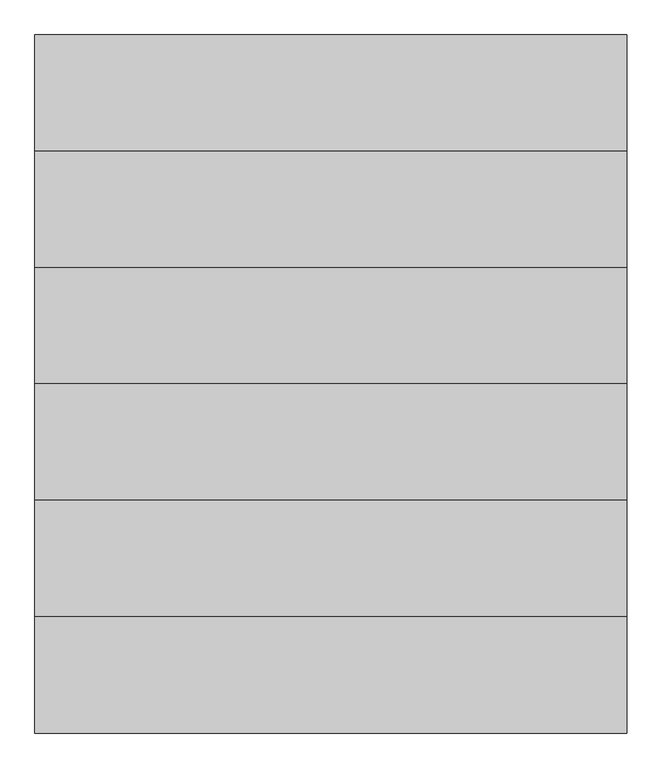
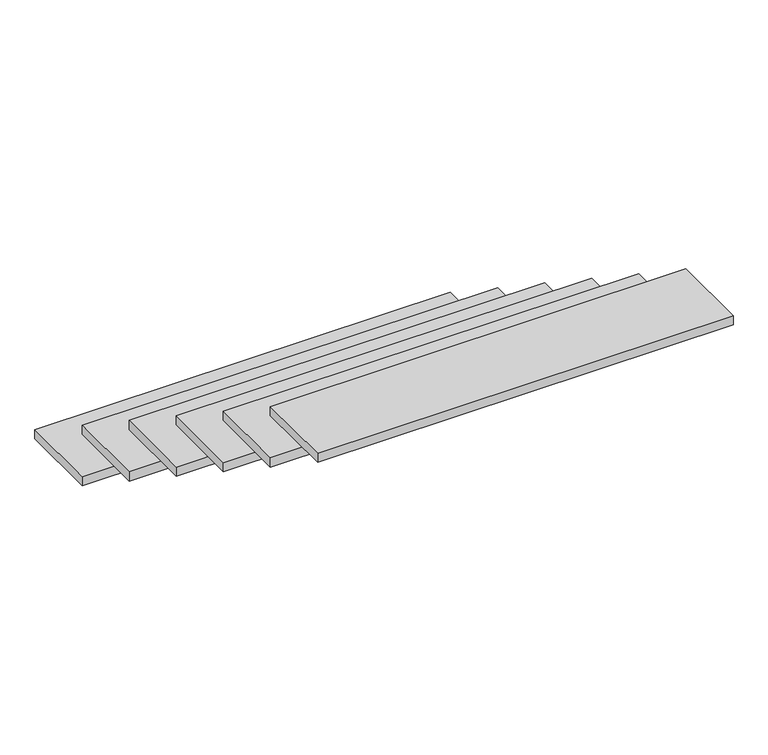
"""IFC4 building model written with IfcOpenShell, lengths in millimetres: stair flight geometry."""

from ifc_helpers import new_model, si_unit, frame, origin, place, context, project, spatial, polyline, outline, extrude, source, transform, mapped, element, save


def stair_flight_8ae47249(model_context):
    return source(origin(), model_context, "Body", "SweptSolid", [
        extrude(outline(polyline([(13552.1845799, 2149.5208589), (12177.1845799, 2149.5208589), (12177.1845799, 2419.5208589), (13552.1845799, 2419.5208589), (13552.1845799, 2149.5208589)])), frame((0.0, 0.0, 7817.9618634), z_axis=(0.0, 0.0, 1.0), x_axis=(1.0, 0.0, 0.0)), (0.0, 0.0, 1.0), 32.0),
        extrude(outline(polyline([(13552.1845799, 1879.5208589), (12177.1845799, 1879.5208589), (12177.1845799, 2149.5208589), (13552.1845799, 2149.5208589), (13552.1845799, 1879.5208589)])), frame((0.0, 0.0, 7997.9618634), z_axis=(0.0, 0.0, 1.0), x_axis=(1.0, 0.0, 0.0)), (0.0, 0.0, 1.0), 32.0),
        extrude(outline(polyline([(13552.1845799, 1609.5208589), (12177.1845799, 1609.5208589), (12177.1845799, 1879.5208589), (13552.1845799, 1879.5208589), (13552.1845799, 1609.5208589)])), frame((0.0, 0.0, 8177.9618634), z_axis=(0.0, 0.0, 1.0), x_axis=(1.0, 0.0, 0.0)), (0.0, 0.0, 1.0), 32.0),
        extrude(outline(polyline([(13552.1845799, 1339.5208589), (12177.1845799, 1339.5208589), (12177.1845799, 1609.5208589), (13552.1845799, 1609.5208589), (13552.1845799, 1339.5208589)])), frame((0.0, 0.0, 8357.9618634), z_axis=(0.0, 0.0, 1.0), x_axis=(1.0, 0.0, 0.0)), (0.0, 0.0, 1.0), 32.0),
        extrude(outline(polyline([(13552.1845799, 1069.5208589), (12177.1845799, 1069.5208589), (12177.1845799, 1339.5208589), (13552.1845799, 1339.5208589), (13552.1845799, 1069.5208589)])), frame((0.0, 0.0, 8537.9618634), z_axis=(0.0, 0.0, 1.0), x_axis=(1.0, 0.0, 0.0)), (0.0, 0.0, 1.0), 32.0),
        extrude(outline(polyline([(13552.1845799, 799.5208589), (12177.1845799, 799.5208589), (12177.1845799, 1069.5208589), (13552.1845799, 1069.5208589), (13552.1845799, 799.5208589)])), frame((0.0, 0.0, 8717.9618634), z_axis=(0.0, 0.0, 1.0), x_axis=(1.0, 0.0, 0.0)), (0.0, 0.0, 1.0), 32.0),
    ])


if __name__ == "__main__":
    model = new_model("IFC4")
    model_context = context("Model", 3, world=origin())
    ifc_project = project(units=[si_unit("LENGTHUNIT", "METRE", prefix="MILLI")], contexts=[model_context])
    site = spatial("IfcSite", under=ifc_project)
    building = spatial("IfcBuilding", under=site)
    placement = place(None, origin())
    stair_flight_shape = stair_flight_8ae47249(model_context)
    element("IfcStairFlight", 1, at=placement, inside=building, context=model_context, shape_type="MappedRepresentation", body=[
        mapped(stair_flight_shape, transform((0.0, 0.0, 0.0), x_axis=(1.0, 0.0, 0.0), y_axis=(0.0, 1.0, 0.0), z_axis=(0.0, 0.0, 1.0))),
    ])
    save(model, "model.ifc")
